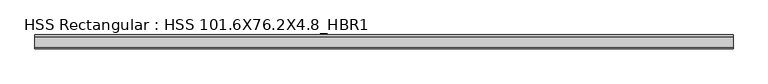
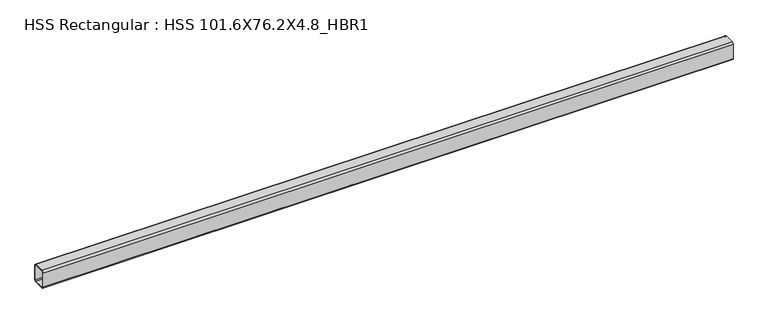
"""IFC4 building model written with IfcOpenShell, lengths in millimetres: beam geometry, HSS Rectangular : HSS 101.6X76.2X4.8_HBR1."""

from ifc_helpers import new_model, si_unit, point, frame, frame_2d, origin, place, context, project, spatial, polyline, circle_curve, trimmed, segment, composite_curve, outline, extrude, source, transform, mapped, element, save


def hss_rectangular_hss_101_6x76_2x4_8_hbr1_00ff1198(model_context):
    return source(origin(), model_context, "Body", "SweptSolid", [
        extrude(outline(composite_curve([segment(polyline([(38.1, 41.275), (38.1, -41.275)]), True, "CONTINUOUS"), segment(trimmed(circle_curve(frame_2d((28.575, -41.275)), 9.525), [point((38.1, -41.275))], [point((28.575, -50.8))], False, "CARTESIAN"), True, "CONTINUOUS"), segment(polyline([(28.575, -50.8), (-28.575, -50.8)]), True, "CONTINUOUS"), segment(trimmed(circle_curve(frame_2d((-28.575, -41.275)), 9.525), [point((-28.575, -50.8))], [point((-38.1, -41.275))], False, "CARTESIAN"), True, "CONTINUOUS"), segment(polyline([(-38.1, -41.275), (-38.1, 41.275)]), True, "CONTINUOUS"), segment(trimmed(circle_curve(frame_2d((-28.575, 41.275)), 9.525), [point((-38.1, 41.275))], [point((-28.575, 50.8))], False, "CARTESIAN"), True, "CONTINUOUS"), segment(polyline([(-28.575, 50.8), (28.575, 50.8)]), True, "CONTINUOUS"), segment(trimmed(circle_curve(frame_2d((28.575, 41.275)), 9.525), [point((28.575, 50.8))], [point((38.1, 41.275))], False, "CARTESIAN"), True, "CONTINUOUS")], self_intersect=False), holes=[composite_curve([segment(trimmed(circle_curve(frame_2d((-28.575, 41.275)), 4.7625), [point((-28.575, 46.0375))], [point((-33.3375, 41.275))], True, "CARTESIAN"), True, "CONTINUOUS"), segment(polyline([(-33.3375, 41.275), (-33.3375, -41.275)]), True, "CONTINUOUS"), segment(trimmed(circle_curve(frame_2d((-28.575, -41.275)), 4.7625), [point((-33.3375, -41.275))], [point((-28.575, -46.0375))], True, "CARTESIAN"), True, "CONTINUOUS"), segment(polyline([(-28.575, -46.0375), (28.575, -46.0375)]), True, "CONTINUOUS"), segment(trimmed(circle_curve(frame_2d((28.575, -41.275)), 4.7625), [point((28.575, -46.0375))], [point((33.3375, -41.275))], True, "CARTESIAN"), True, "CONTINUOUS"), segment(polyline([(33.3375, -41.275), (33.3375, 41.275)]), True, "CONTINUOUS"), segment(trimmed(circle_curve(frame_2d((28.575, 41.275)), 4.7625), [point((33.3375, 41.275))], [point((28.575, 46.0375))], True, "CARTESIAN"), True, "CONTINUOUS"), segment(polyline([(28.575, 46.0375), (-28.575, 46.0375)]), True, "CONTINUOUS")], self_intersect=False)]), frame((-1928.4431192, 0.0, 0.0), z_axis=(1.0, 0.0, 0.0), x_axis=(0.0, 1.0, 0.0)), (0.0, 0.0, 1.0), 3814.4286584),
    ])


if __name__ == "__main__":
    model = new_model("IFC4")
    model_context = context("Model", 3, world=origin())
    ifc_project = project(units=[si_unit("LENGTHUNIT", "METRE", prefix="MILLI")], contexts=[model_context])
    site = spatial("IfcSite", under=ifc_project)
    building = spatial("IfcBuilding", under=site)
    placement = place(None, origin())
    hss_rectangular_hss_101_6x76_2x4_8_hbr1_shape = hss_rectangular_hss_101_6x76_2x4_8_hbr1_00ff1198(model_context)
    element("IfcBeam", 1, ObjectType="HSS Rectangular : HSS 101.6X76.2X4.8_HBR1", at=placement, inside=building, context=model_context, shape_type="MappedRepresentation", body=[
        mapped(hss_rectangular_hss_101_6x76_2x4_8_hbr1_shape, transform((0.0, 0.0, 0.0), x_axis=(1.0, 0.0, 0.0), y_axis=(0.0, 1.0, 0.0), z_axis=(0.0, 0.0, 1.0))),
    ])
    save(model, "model.ifc")

# Revit data of these elements
# Project information
#   Project Status = "Project Status"
#   Client Name = "현대엔지니어링"
#   Project Address = "서울시 종로구 율곡로 75(계동)"
#   Project Number = "-"
# Type "HSS Rectangular : HSS 101.6X76.2X4.8_HBR1"
#   Section Name Key = "HSS 4X3X3/16"
#   Assembly Code = "B10"
#   Width = 7.62 cm
#   Wall Nominal Thickness = 0.4763 cm
#   Wall Design Thickness = 0.442 cm
#   Torsional Moment of Inertia = 260.561 cm⁴
#   Torsional Modulus = 61.2876 cm³
#   Section Area = 14.4516 cm²
#   Plastic Modulus weak axis = 40.3122 cm³
#   Plastic Modulus strong axis = 49.1612 cm³
#   Perimeter = 0.881482 m²/m
#   Outer Fillet = 0.9525 cm
#   Nominal Weight = 12.1285 kgf/m
#   Moment of Inertia weak axis = 131.529 cm⁴
#   Moment of Inertia strong axis = 205.202 cm⁴
#   Inner Fillet = 0.4763 cm
#   Height = 10.16 cm
#   Elastic Modulus weak axis = 34.4128 cm³
#   Elastic Modulus strong axis = 40.476 cm³
#   Centroid Vertical = 5.08 cm
#   Centroid Horizontal = 3.81 cm
#   Length [instance default] = 1524 mm
#   Structural Material [instance default] = Steel ASTM A500, Grade B, Rectangular and Square
#   Principal Axes Angle = 0
# Element 1 (IfcBeam, "HSS Rectangular : HSS 101.6X76.2X4.8_HBR1")
#   Structural Material = Steel ASTM A992
#   Materials on its faces: "Steel ASTM A992"
# Materials
#   "Steel ASTM A500, Grade B, Rectangular and Square": class "Metal", colour RGB 199 199 199, transparency 0, Description = "Carbon steel", Cost = 0
#   "Steel ASTM A992": class "Metal", colour RGB 199 199 199, transparency 0, Description = "Structural steel 50ksi", Cost = 0
